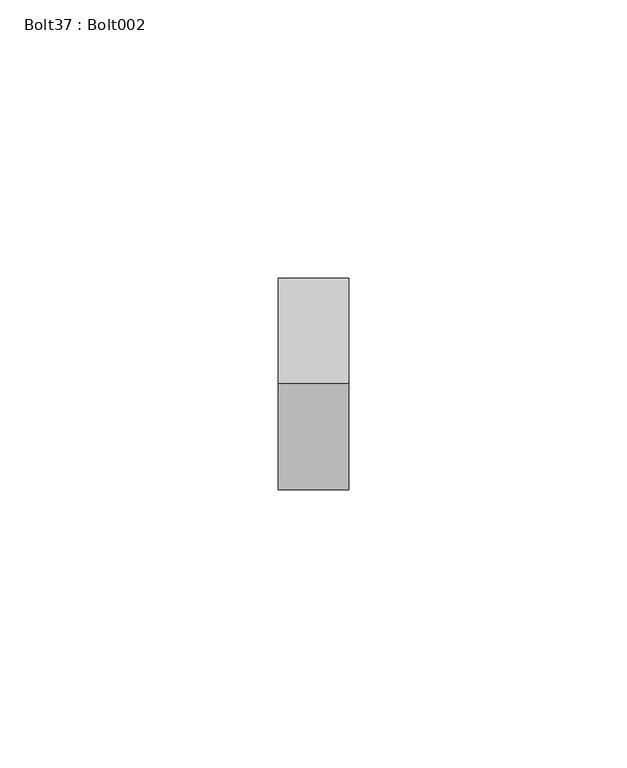
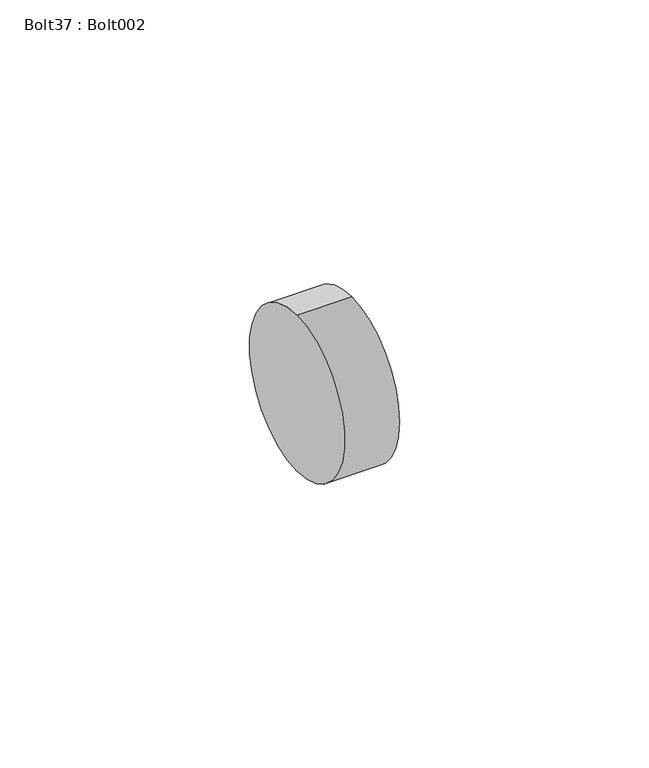
"""IFC4 building model written with IfcOpenShell, lengths in millimetres: proxy geometry, Bolt37 : Bolt002."""

from ifc_helpers import new_model, si_unit, point, frame, frame_2d, origin, place, context, project, spatial, circle_curve, trimmed, segment, composite_curve, outline, extrude, source, transform, mapped, element, save


def bolt37_bolt002_beea302d(model_context):
    return source(origin(), model_context, "Body", "SweptSolid", [
        extrude(outline(composite_curve([segment(trimmed(circle_curve(frame_2d((1985.8304801, 40070.0545241)), 19.05), [point((1985.8304801, 40051.0045241))], [point((1985.8304801, 40089.1045241))], False, "CARTESIAN"), True, "CONTINUOUS"), segment(trimmed(circle_curve(frame_2d((1985.8304801, 40070.0545241)), 19.05), [point((1985.8304801, 40089.1045241))], [point((1985.8304801, 40051.0045241))], False, "CARTESIAN"), True, "CONTINUOUS")], self_intersect=False)), frame((10268.2640809, 0.0, 0.0), z_axis=(1.0, 0.0, 0.0), x_axis=(0.0, 1.0, 0.0)), (0.0, 0.0, 1.0), 12.7),
    ])


if __name__ == "__main__":
    model = new_model("IFC4")
    model_context = context("Model", 3, world=origin())
    ifc_project = project(units=[si_unit("LENGTHUNIT", "METRE", prefix="MILLI")], contexts=[model_context])
    site = spatial("IfcSite", under=ifc_project)
    building = spatial("IfcBuilding", under=site)
    placement = place(None, origin())
    bolt37_bolt002_shape = bolt37_bolt002_beea302d(model_context)
    element("IfcBuildingElementProxy", 1, Name="Bolt37 : Bolt002", ObjectType="Bolt37 : Bolt002", at=placement, inside=building, context=model_context, shape_type="MappedRepresentation", body=[
        mapped(bolt37_bolt002_shape, transform((0.0, 0.0, 0.0), x_axis=(1.0, 0.0, 0.0), y_axis=(0.0, 1.0, 0.0), z_axis=(0.0, 0.0, 1.0))),
    ])
    save(model, "model.ifc")

# Revit data of these elements
# Type "Bolt37 : Bolt002"
#   NameOverride = "Bolt002"
# Element 1 (IfcBuildingElementProxy, "Bolt37 : Bolt002")
#   Materials on its faces: "STEEL ANGLE AND ANCHOR BOLT (SEE STRUCT. DWGS)"
# Materials
#   "STEEL ANGLE AND ANCHOR BOLT (SEE STRUCT. DWGS)": class "Unassigned", colour RGB 128 128 128, transparency 0, Cost = 0
